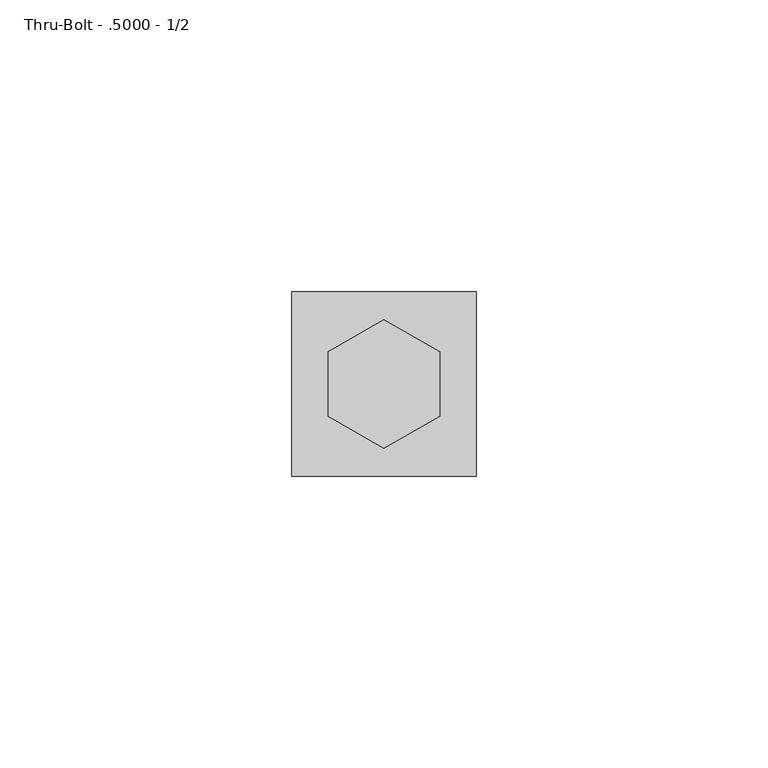
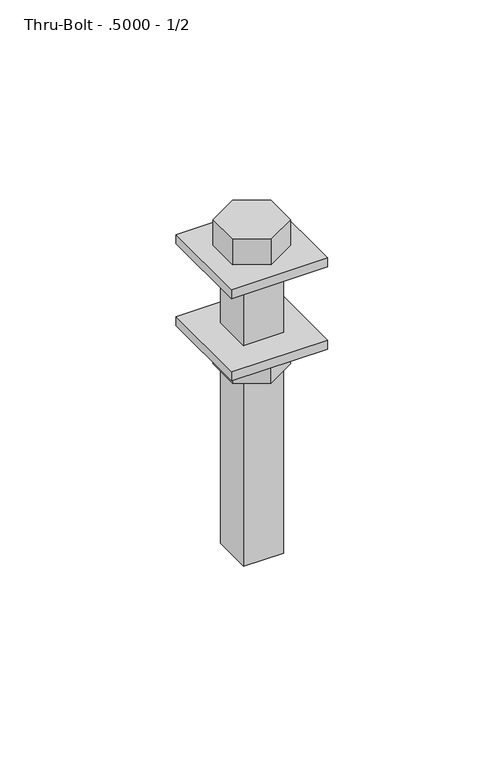
"""IFC4 building model written with IfcOpenShell, lengths in millimetres: fastener geometry, 060523 - W_P_C - Fastenings - Generic - SQUARE : Thru-Bolt - .5000 - 1/2."""

from ifc_helpers import new_model, si_unit, frame, origin, origin_with_axes, place, context, project, spatial, polyline, outline, extrude, source, transform, mapped, element, save


def thru_bolt_5000_1_2_b29ce19b(model_context):
    return source(origin(), model_context, "Body", "SweptSolid", [
        extrude(outline(polyline([(-15.7757813, -15.7757813), (-15.7757813, 15.7757812), (15.7757812, 15.7757812), (15.7757812, -15.7757813), (-15.7757813, -15.7757813)])), origin_with_axes(), (0.0, 0.0, 1.0), 3.0757812),
        extrude(outline(polyline([(-15.7757813, -15.7757813), (-15.7757813, 15.7757812), (15.7757812, 15.7757812), (15.7757812, -15.7757813), (-15.7757813, -15.7757813)])), frame((0.0, 0.0, -28.4757813), z_axis=(0.0, 0.0, 1.0), x_axis=(1.0, 0.0, 0.0)), (0.0, 0.0, 1.0), 3.0757812),
        extrude(outline(polyline([(-9.525, -5.4992613), (-9.525, 5.4992613), (0.0, 10.9985226), (9.525, 5.4992613), (9.525, -5.4992613), (0.0, -10.9985226), (-9.525, -5.4992613)])), frame((0.0, 0.0, -37.703125), z_axis=(0.0, 0.0, 1.0), x_axis=(1.0, 0.0, 0.0)), (0.0, 0.0, 1.0), 9.2273437),
        extrude(outline(polyline([(-9.525, 5.4992613), (0.0, 10.9985226), (9.525, 5.4992613), (9.525, -5.4992613), (0.0, -10.9985226), (-9.525, -5.4992613), (-9.525, 5.4992613)])), frame((0.0, 0.0, 3.0757813), z_axis=(0.0, 0.0, 1.0), x_axis=(1.0, 0.0, 0.0)), (0.0, 0.0, 1.0), 9.2273437),
        extrude(outline(polyline([(-6.5484375, 6.5484375), (6.5484375, 6.5484375), (6.5484375, -6.5484375), (-6.5484375, -6.5484375), (-6.5484375, 6.5484375)])), frame((0.0, 0.0, -101.6), z_axis=(0.0, 0.0, 1.0), x_axis=(1.0, 0.0, 0.0)), (0.0, 0.0, 1.0), 104.6757812),
    ])


if __name__ == "__main__":
    model = new_model("IFC4")
    model_context = context("Model", 3, world=origin())
    ifc_project = project(units=[si_unit("LENGTHUNIT", "METRE", prefix="MILLI")], contexts=[model_context])
    site = spatial("IfcSite", under=ifc_project)
    building = spatial("IfcBuilding", under=site)
    placement = place(None, origin())
    thru_bolt_5000_1_2_shape = thru_bolt_5000_1_2_b29ce19b(model_context)
    element("IfcFastener", 1, ObjectType="060523 - W_P_C - Fastenings - Generic - SQUARE : Thru-Bolt - .5000 - 1/2", at=placement, inside=building, context=model_context, shape_type="MappedRepresentation", body=[
        mapped(thru_bolt_5000_1_2_shape, transform((0.0, 0.0, 0.0), x_axis=(1.0, 0.0, 0.0), y_axis=(0.0, 1.0, 0.0), z_axis=(0.0, 0.0, 1.0))),
    ])
    save(model, "model.ifc")

# Revit data of these elements
# Type "060523 - W_P_C - Fastenings - Generic - SQUARE : Thru-Bolt - .5000 - 1/2"
#   Washer_Thickness = 0' - 0 31/256"
#   Washer Radius = 0' - 0 159/256"
#   Washer Offset - Head = 0' - 0 31/256"
#   Washer Offset = 0' - 0 31/256"
#   Thickness_of_Substrate [instance default] = 0' - 1"
#   Side = 0' - 0 111/256"
#   Radius = 0' - 0 33/128"
#   Length [instance default] = 0' - 4"
#   Head Size = 0' - 0 3/4"
#   Head Radius = 0' - 0 3/8"
#   Head Height = 0' - 0 93/256"
#   Double Diameter = 0' - 1 1/32"
#   Diameter = 0' - 0 33/64"
#   Default Elevation = 4' - 0"
#   Washer_Nut_Visibility = yes
#   Washer_Head_Visibility = yes
#   Round_Head_Visibility = no
#   Point Visibility = no
#   Nut_Visibility = yes
#   Hex_Head_Visiblilty = yes
#   Washer Material = none
#   Bolt Material (Size) = AT SILL - FASTENER AT 24" O.C.
# Element 1 (IfcFastener, "060523 - W_P_C - Fastenings - Generic - SQUARE : Thru-Bolt - .5000 - 1/2")
#   Materials on its faces: "AT SILL - FASTENER AT 24\" O.C."
# Materials
#   "AT SILL - FASTENER AT 24\" O.C.": class "Generic", colour RGB 120 120 120, transparency 0, Cost = 0
